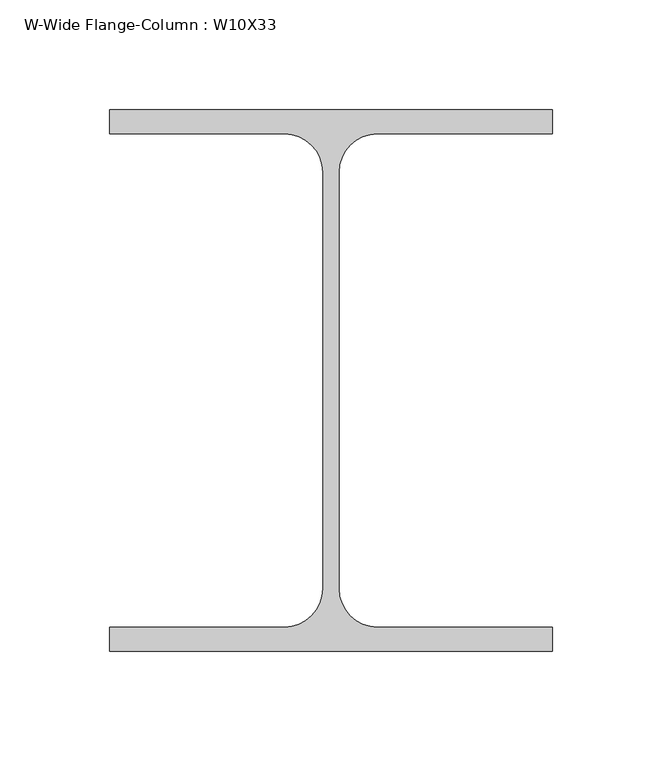
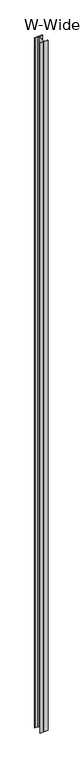
"""IFC4 building model written with IfcOpenShell, lengths in millimetres: column geometry, W-Wide Flange-Column : W10X33."""

from ifc_helpers import new_model, si_unit, point, frame, frame_2d, origin, place, context, project, spatial, polyline, circle_curve, trimmed, segment, composite_curve, outline, extrude, source, transform, mapped, element, save


def w_wide_flange_column_w10x33_f3eae173(model_context):
    return source(origin(), model_context, "Body", "SweptSolid", [
        extrude(outline(composite_curve([segment(polyline([(101.092, 123.571), (101.092, 112.522), (21.209, 112.522)]), True, "CONTINUOUS"), segment(trimmed(circle_curve(frame_2d((21.209, 94.996)), 17.526), [point((21.209, 112.522))], [point((3.683, 94.996))], True, "CARTESIAN"), True, "CONTINUOUS"), segment(polyline([(3.683, 94.996), (3.683, -94.996)]), True, "CONTINUOUS"), segment(trimmed(circle_curve(frame_2d((21.209, -94.996)), 17.526), [point((3.683, -94.996))], [point((21.209, -112.522))], True, "CARTESIAN"), True, "CONTINUOUS"), segment(polyline([(21.209, -112.522), (101.092, -112.522), (101.092, -123.571), (-101.092, -123.571), (-101.092, -112.522), (-21.209, -112.522)]), True, "CONTINUOUS"), segment(trimmed(circle_curve(frame_2d((-21.209, -94.996)), 17.526), [point((-21.209, -112.522))], [point((-3.683, -94.996))], True, "CARTESIAN"), True, "CONTINUOUS"), segment(polyline([(-3.683, -94.996), (-3.683, 94.996)]), True, "CONTINUOUS"), segment(trimmed(circle_curve(frame_2d((-21.209, 94.996)), 17.526), [point((-3.683, 94.996))], [point((-21.209, 112.522))], True, "CARTESIAN"), True, "CONTINUOUS"), segment(polyline([(-21.209, 112.522), (-101.092, 112.522), (-101.092, 123.571), (101.092, 123.571)]), True, "CONTINUOUS")], self_intersect=False)), frame((0.0, 0.0, 8756.65), z_axis=(0.0, 0.0, 1.0), x_axis=(1.0, 0.0, 0.0)), (0.0, 0.0, 1.0), 18827.75),
    ])


if __name__ == "__main__":
    model = new_model("IFC4")
    model_context = context("Model", 3, world=origin())
    ifc_project = project(units=[si_unit("LENGTHUNIT", "METRE", prefix="MILLI")], contexts=[model_context])
    site = spatial("IfcSite", under=ifc_project)
    building = spatial("IfcBuilding", under=site)
    placement = place(None, origin())
    w_wide_flange_column_w10x33_shape = w_wide_flange_column_w10x33_f3eae173(model_context)
    element("IfcColumn", 1, ObjectType="W-Wide Flange-Column : W10X33", at=placement, inside=building, context=model_context, shape_type="MappedRepresentation", body=[
        mapped(w_wide_flange_column_w10x33_shape, transform((0.0, 0.0, 0.0), x_axis=(1.0, 0.0, 0.0), y_axis=(0.0, 1.0, 0.0), z_axis=(0.0, 0.0, 1.0))),
    ])
    save(model, "model.ifc")

# Revit data of these elements
# Type "W-Wide Flange-Column : W10X33"
#   Assembly Code = "B10"
#   W = 33
#   bf = 0' - 7.96"
#   d = 0' - 9.73"
#   k = 0' - 1 1/8"
#   kr = 0' - 0.69"
#   tf = 0' - 0.435"
#   tw = 0' - 0.29"
#   A = 0.0674306 SF
#   Structural Material [instance default] = Steel ASTM A992
# Element 1 (IfcColumn, "W-Wide Flange-Column : W10X33")
#   Materials on its faces: "Steel ASTM A992"
# Materials
#   "Steel ASTM A992": class "Metal", colour RGB 199 199 199, transparency 0, Description = "Structural steel 50ksi", Cost = 0
